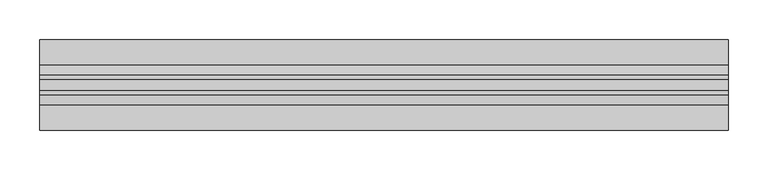
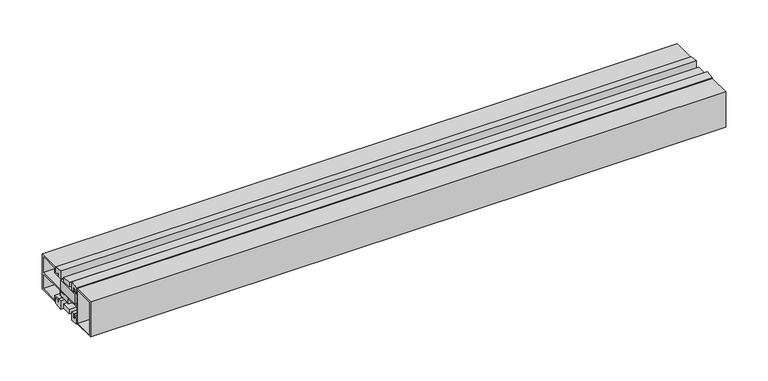
"""IFC4 building model written with IfcOpenShell, lengths in millimetres: proxy geometry, Generic Models 3:Generic Models 1:3:Generic Models 1:3 : Generic Models 3:Generic Models 1:300625:336034:Generic Models 1:3:Generic Models 1:3 : Generic Models 3:Generic Models 1:300625:336034 : Generic Models 3:Generic Models 1:3:Generic Models 1:3 : Generic Models 3:Generic Models 1:300625:336034:3 : Generic Models 3:Generic Models 1:3:Generic Models 1:3 : Generic Models 3:Generic Models 1:300625:336034:Generic Models 1:3:Generic Models 1:3 : Generic Models 3:Generic Models 1:300625:336034 : Generic Models 3:Generic Models 1:3:Generic Models 1:3 : Generic Models 3:Generic Models 1:300625:336034:301191."""

from ifc_helpers import new_model, si_unit, frame, origin, place, context, project, spatial, polyline, outline, extrude, source, transform, mapped, element, save


def generic_models_d537cfb8(model_context):
    return source(origin(), model_context, "Body", "SweptSolid", [
        extrude(outline(polyline([(570395.4867239, -579054.6832724), (570395.4867239, -579067.3832724), (569527.1242239, -579067.3832724), (569527.1242239, -579054.6832724), (570395.4867239, -579054.6832724)])), frame((0.0, 0.0, 2441.2521298), z_axis=(0.0, 0.0, 1.0), x_axis=(1.0, 0.0, 0.0)), (0.0, 0.0, 1.0), 6.3435484),
        extrude(outline(polyline([(-579086.0195091, 2437.3831629), (-579086.0195091, 2445.2228723), (-579081.7214373, 2445.2228723), (-579081.7214373, 2442.2790126), (-579078.8757591, 2442.2790126), (-579078.8757591, 2447.9925532), (-579074.1217032, 2447.9925532), (-579074.1217032, 2435.9222961), (-579086.0195091, 2437.3831629)])), frame((569527.1242239, 0.0, 0.0), z_axis=(1.0, 0.0, 0.0), x_axis=(0.0, 1.0, 0.0)), (0.0, 0.0, 1.0), 868.3625),
        extrude(outline(polyline([(-579043.1907857, 2442.2790126), (-579040.3451075, 2442.2790126), (-579040.3451075, 2445.2228723), (-579036.0470357, 2445.2228723), (-579036.0470357, 2437.3831629), (-579047.9448415, 2435.9222961), (-579047.9448415, 2447.9925532), (-579043.1907857, 2447.9925532), (-579043.1907857, 2442.2790126)])), frame((569527.1242239, 0.0, 0.0), z_axis=(1.0, 0.0, 0.0), x_axis=(0.0, 1.0, 0.0)), (0.0, 0.0, 1.0), 868.3625),
        extrude(outline(polyline([(570395.4867239, -579047.2017564), (570395.4867239, -579080.4885915), (569527.1242239, -579080.4885915), (569527.1242239, -579047.2017564), (570395.4867239, -579047.2017564)])), frame((0.0, 0.0, 2463.7831117), z_axis=(0.0, 0.0, 1.0), x_axis=(1.0, 0.0, 0.0)), (0.0, 0.0, 1.0), 14.2115027),
        extrude(outline(polyline([(570395.4867239, -579047.8857325), (570395.4867239, -579063.9971687), (569527.1242239, -579063.9971687), (569527.1242239, -579047.8857325), (570395.4867239, -579047.8857325)])), frame((0.0, 0.0, 2455.803391), z_axis=(0.0, 0.0, 1.0), x_axis=(1.0, 0.0, 0.0)), (0.0, 0.0, 1.0), 6.0797872),
        extrude(outline(polyline([(570395.4867239, -579054.6832724), (570395.4867239, -579067.3832724), (569527.1242239, -579067.3832724), (569527.1242239, -579054.6832724), (570395.4867239, -579054.6832724)])), frame((0.0, 0.0, 2479.9705452), z_axis=(0.0, 0.0, 1.0), x_axis=(1.0, 0.0, 0.0)), (0.0, 0.0, 1.0), 6.3435484),
        extrude(outline(polyline([(-579078.8757591, 2485.2872108), (-579081.7214373, 2485.2872108), (-579081.7214373, 2482.3433511), (-579086.0195091, 2482.3433511), (-579086.0195091, 2490.1830605), (-579074.1217032, 2491.6439273), (-579074.1217032, 2479.5736702), (-579078.8757591, 2479.5736702), (-579078.8757591, 2485.2872108)])), frame((569527.1242239, 0.0, 0.0), z_axis=(1.0, 0.0, 0.0), x_axis=(0.0, 1.0, 0.0)), (0.0, 0.0, 1.0), 868.3625),
        extrude(outline(polyline([(-579036.0470357, 2490.1830605), (-579036.0470357, 2482.3433511), (-579040.3451075, 2482.3433511), (-579040.3451075, 2485.2872108), (-579043.1907857, 2485.2872108), (-579043.1907857, 2479.5736702), (-579047.9448415, 2479.5736702), (-579047.9448415, 2491.6439273), (-579036.0470357, 2490.1830605)])), frame((569527.1242239, 0.0, 0.0), z_axis=(1.0, 0.0, 0.0), x_axis=(0.0, 1.0, 0.0)), (0.0, 0.0, 1.0), 868.3625),
        extrude(outline(polyline([(-579118.1663841, 2438.4), (-579118.1663841, 2489.1662234), (-579086.4163841, 2489.1662234), (-579086.4163841, 2481.9464761), (-579081.3245623, 2481.9464761), (-579081.3245623, 2484.8903358), (-579079.2726341, 2484.8903358), (-579079.2726341, 2479.9705452), (-579086.4163841, 2479.9705452), (-579086.4163841, 2463.7831117), (-579059.1333389, 2463.7831117), (-579059.1333389, 2461.8831782), (-579063.9971687, 2461.8831782), (-579063.9971687, 2455.803391), (-579059.1333389, 2455.803391), (-579059.1333389, 2454.5114362), (-579065.8971022, 2454.5114362), (-579065.8971022, 2461.8831782), (-579086.4163841, 2461.8831782), (-579086.4163841, 2447.6716755), (-579079.2726341, 2447.6716755), (-579079.2726341, 2443.1005159), (-579081.3245623, 2443.1005159), (-579081.3245623, 2445.6197473), (-579086.4163841, 2445.6197473), (-579086.4163841, 2438.4), (-579118.1663841, 2438.4)]), holes=[polyline([(-579088.3163176, 2487.2662899), (-579115.6584719, 2487.2662899), (-579115.6584719, 2440.2999335), (-579088.3163176, 2440.2999335), (-579088.3163176, 2487.2662899)])]), frame((569527.1242239, 0.0, 0.0), z_axis=(1.0, 0.0, 0.0), x_axis=(0.0, 1.0, 0.0)), (0.0, 0.0, 1.0), 868.3625),
        extrude(outline(polyline([(-579040.7419825, 2484.8903358), (-579040.7419825, 2481.9464761), (-579035.6501607, 2481.9464761), (-579035.6501607, 2489.1662234), (-579003.8663841, 2489.1662234), (-579003.8663841, 2438.4), (-579035.6501607, 2438.4), (-579035.6501607, 2445.6197473), (-579040.7419825, 2445.6197473), (-579040.7419825, 2443.1005159), (-579042.7939107, 2443.1005159), (-579042.7939107, 2447.6716755), (-579033.7502272, 2447.6716755), (-579033.7502272, 2440.3222126), (-579005.8423149, 2440.3222126), (-579005.8423149, 2461.8831782), (-579045.985799, 2461.8831782), (-579045.985799, 2454.5114362), (-579052.7495623, 2454.5114362), (-579052.7495623, 2455.803391), (-579047.8857325, 2455.803391), (-579047.8857325, 2461.8831782), (-579052.7495623, 2461.8831782), (-579052.7495623, 2463.7831117), (-579005.8423149, 2463.7831117), (-579005.8423149, 2487.2564243), (-579033.7502272, 2487.2564243), (-579033.7502272, 2479.9705452), (-579042.7939107, 2479.9705452), (-579042.7939107, 2484.8903358), (-579040.7419825, 2484.8903358)])), frame((569527.1242239, 0.0, 0.0), z_axis=(1.0, 0.0, 0.0), x_axis=(0.0, 1.0, 0.0)), (0.0, 0.0, 1.0), 868.3625),
    ])


if __name__ == "__main__":
    model = new_model("IFC4")
    model_context = context("Model", 3, world=origin())
    ifc_project = project(units=[si_unit("LENGTHUNIT", "METRE", prefix="MILLI")], contexts=[model_context])
    site = spatial("IfcSite", under=ifc_project)
    building = spatial("IfcBuilding", under=site)
    placement = place(None, origin())
    generic_models_shape = generic_models_d537cfb8(model_context)
    element("IfcBuildingElementProxy", 1, Name="Generic Models 3:Generic Models 1:3:Generic Models 1:3 : Generic Models 3:Generic Models 1:300625:336034:Generic Models 1:3:Generic Models 1:3 : Generic Models 3:Generic Models 1:300625:336034 : Generic Models 3:Generic Models 1:3:Generic Models 1:3 : Generic Models 3:Generic Models 1:300625:336034:3 : Generic Models 3:Generic Models 1:3:Generic Models 1:3 : Generic Models 3:Generic Models 1:300625:336034:Generic Models 1:3:Generic Models 1:3 : Generic Models 3:Generic Models 1:300625:336034 : Generic Models 3:Generic Models 1:3:Generic Models 1:3 : Generic Models 3:Generic Models 1:300625:336034:301191", ObjectType="Generic Models 3:Generic Models 1:3:Generic Models 1:3 : Generic Models 3:Generic Models 1:300625:336034:Generic Models 1:3:Generic Models 1:3 : Generic Models 3:Generic Models 1:300625:336034 : Generic Models 3:Generic Models 1:3:Generic Models 1:3 : Generic Models 3:Generic Models 1:300625:336034:3 : Generic Models 3:Generic Models 1:3:Generic Models 1:3 : Generic Models 3:Generic Models 1:300625:336034:Generic Models 1:3:Generic Models 1:3 : Generic Models 3:Generic Models 1:300625:336034 : Generic Models 3:Generic Models 1:3:Generic Models 1:3 : Generic Models 3:Generic Models 1:300625:336034:301191", at=placement, inside=building, context=model_context, shape_type="MappedRepresentation", body=[
        mapped(generic_models_shape, transform((0.0, 0.0, 0.0), x_axis=(1.0, 0.0, 0.0), y_axis=(0.0, 1.0, 0.0), z_axis=(0.0, 0.0, 1.0))),
    ])
    save(model, "model.ifc")

# Revit data of these elements
# Type "Generic Models 3:Generic Models 1:3:Generic Models 1:3 : Generic Models 3:Generic Models 1:300625:336034:Generic Models 1:3:Generic Models 1:3 : Generic Models 3:Generic Models 1:300625:336034 : Generic Models 3:Generic Models 1:3:Generic Models 1:3 : Generic Models 3:Generic Models 1:300625:336034:3 : Generic Models 3:Generic Models 1:3:Generic Models 1:3 : Generic Models 3:Generic Models 1:300625:336034:Generic Models 1:3:Generic Models 1:3 : Generic Models 3:Generic Models 1:300625:336034 : Generic Models 3:Generic Models 1:3:Generic Models 1:3 : Generic Models 3:Generic Models 1:300625:336034:301191"
#   NameOverride = "Generic Models 3:Generic Models 1:3:Generic Models 1:3 : Generic Models 3:Generic Models 1:300625:336034:Generic Models 1:3:Generic Models 1:3 : Generic Models 3:Generic Models 1:300625:336034 : Generic Models 3:Generic Models 1:3:Generic Models 1:3 : Generic Models 3:Generic Models 1:300625:336034:301191"
#   ObjectTypeOverride = "Generic Models 1:3:Generic Models 1:3 : Generic Models 3:Generic Models 1:300625:336034 : Generic Models 3:Generic Models 1:3:Generic Models 1:3 : Generic Models 3:Generic Models 1:300625:336034"
#   Reference = "Generic Models 1"
#   Tag = "301191"
# Element 1 (IfcBuildingElementProxy, "Generic Models 3:Generic Models 1:3:Generic Models 1:3 : Generic Models 3:Generic Models 1:300625:336034:Generic Models 1:3:Generic Models 1:3 : Generic Models 3:Generic Models 1:300625:336034 : Generic Models 3:Generic Models 1:3:Generic Models 1:3 : Generic Models 3:Generic Models 1:300625:336034:3 : Generic Models 3:Generic Models 1:3:Generic Models 1:3 : Generic Models 3:Generic Models 1:300625:336034:Generic Models 1:3:Generic Models 1:3 : Generic Models 3:Generic Models 1:300625:336034 : Generic Models 3:Generic Models 1:3:Generic Models 1:3 : Generic Models 3:Generic Models 1:300625:336034:301191")
#   Materials on its faces: "THERMAL BROKEN ALUMINUM STOREFRONT"
# Materials
#   "THERMAL BROKEN ALUMINUM STOREFRONT": class "Unassigned", colour RGB 244 244 244, transparency 0, Cost = 0
